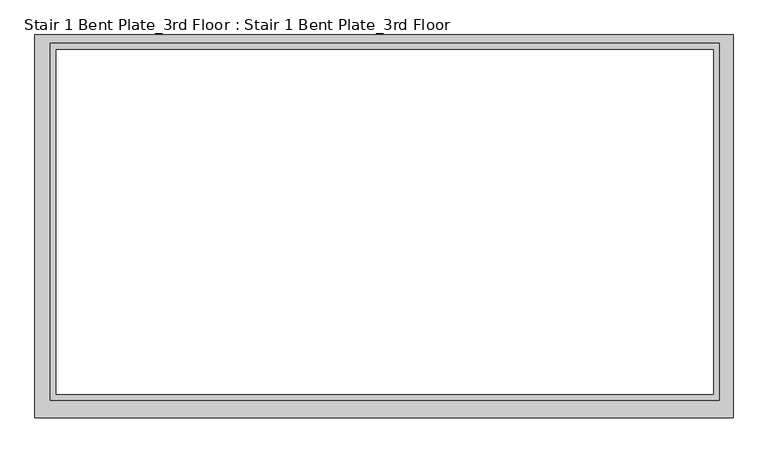
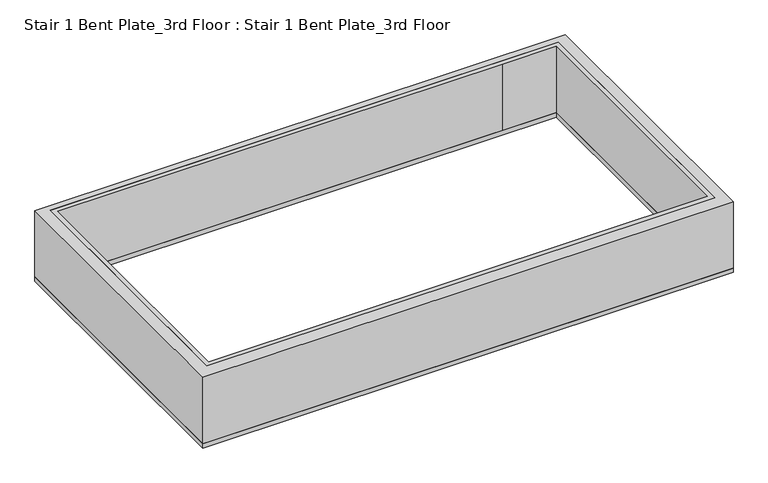
"""IFC4 building model written with IfcOpenShell, lengths in millimetres: proxy geometry, Stair 1 Bent Plate_3rd Floor : Stair 1 Bent Plate_3rd Floor."""

from ifc_helpers import new_model, si_unit, frame, origin, origin_with_axes, place, context, project, spatial, polyline, outline, extrude, source, transform, mapped, element, save


def stair_1_bent_plate_3rd_floor_stair_1_bent_plate_3rd_floor_ed8e0977(model_context):
    return source(origin(), model_context, "Body", "SweptSolid", [
        extrude(outline(polyline([(-279.4, -750.8875), (-279.4, 39.7358273), (1162.05, 39.7358273), (1162.05, -750.8875), (-279.4, -750.8875)]), holes=[polyline([(1133.475, 22.225), (-247.65, 22.225), (-247.65, -714.375), (1133.475, -714.375), (1133.475, 22.225)])]), frame((0.0, 0.0, 12.7), z_axis=(0.0, 0.0, 1.0), x_axis=(1.0, 0.0, 0.0)), (0.0, 0.0, 1.0), 190.5),
        extrude(outline(polyline([(1162.05, -750.8875), (-279.4, -750.8875), (-279.4, 39.7358273), (1162.05, 39.7358273), (1162.05, -750.8875)]), holes=[polyline([(-234.95, 9.525), (-234.95, -701.675), (1120.775, -701.675), (1120.775, 9.525), (-234.95, 9.525)])]), origin_with_axes(), (0.0, 0.0, 1.0), 12.7),
        extrude(outline(polyline([(1133.475, 22.225), (1133.475, -714.375), (-247.65, -714.375), (-247.65, 22.225), (1133.475, 22.225)]), holes=[polyline([(-234.95, -701.675), (1120.775, -701.675), (1120.775, 9.525), (974.725, 9.525), (-234.95, 9.525), (-234.95, -190.5), (-234.95, -701.675)])]), origin_with_axes(), (0.0, 0.0, 1.0), 203.2),
    ])


if __name__ == "__main__":
    model = new_model("IFC4")
    model_context = context("Model", 3, world=origin())
    ifc_project = project(units=[si_unit("LENGTHUNIT", "METRE", prefix="MILLI")], contexts=[model_context])
    site = spatial("IfcSite", under=ifc_project)
    building = spatial("IfcBuilding", under=site)
    placement = place(None, origin())
    stair_1_bent_plate_3rd_floor_stair_1_bent_plate_3rd_floor_shape = stair_1_bent_plate_3rd_floor_stair_1_bent_plate_3rd_floor_ed8e0977(model_context)
    element("IfcBuildingElementProxy", 1, Name="Stair 1 Bent Plate_3rd Floor : Stair 1 Bent Plate_3rd Floor", ObjectType="Stair 1 Bent Plate_3rd Floor : Stair 1 Bent Plate_3rd Floor", at=placement, inside=building, context=model_context, shape_type="MappedRepresentation", body=[
        mapped(stair_1_bent_plate_3rd_floor_stair_1_bent_plate_3rd_floor_shape, transform((0.0, 0.0, 0.0), x_axis=(1.0, 0.0, 0.0), y_axis=(0.0, 1.0, 0.0), z_axis=(0.0, 0.0, 1.0))),
    ])
    save(model, "model.ifc")

# Revit data of these elements
# Element 1 (IfcBuildingElementProxy, "Stair 1 Bent Plate_3rd Floor : Stair 1 Bent Plate_3rd Floor")
#   Materials on its faces: "Concrete Infill"
# Materials
#   "Concrete Infill": class "Generic", colour RGB 0 255 0, transparency 0, Cost = 0
